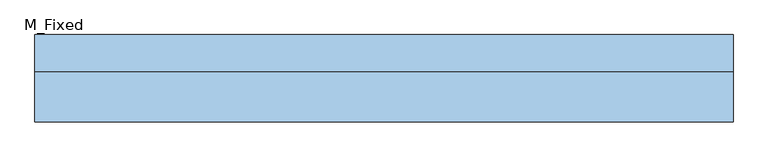
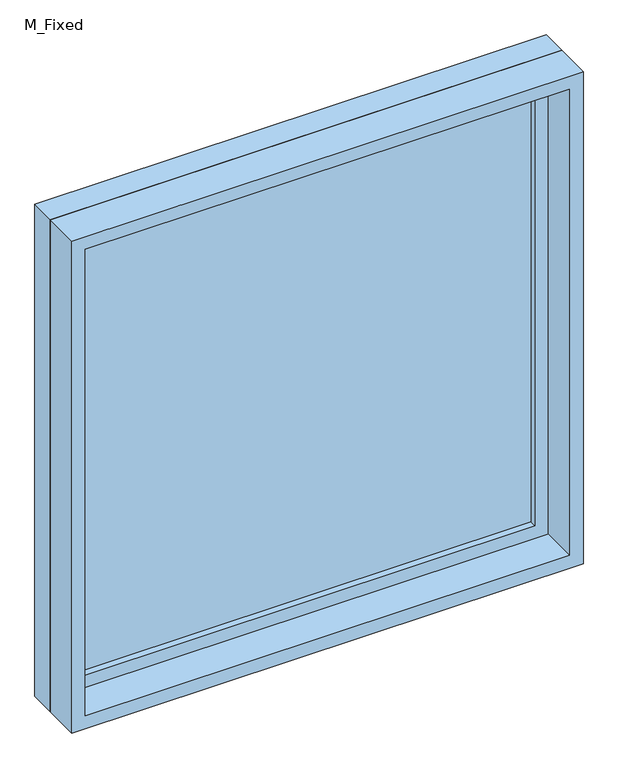
"""IFC4 building model written with IfcOpenShell, lengths in millimetres: window geometry, M_Fixed : W4 1.2 BY 1.2 M."""

from ifc_helpers import new_model, si_unit, frame, origin, place, context, project, spatial, polyline, outline, extrude, source, transform, mapped, element, save


def m_fixed_e389692a(model_context):
    return source(origin(), model_context, "Body", "SweptSolid", [
        extrude(outline(polyline([(-537.0, 53.0), (537.0, 53.0), (537.0, 41.0), (-537.0, 41.0), (-537.0, 53.0)])), frame((0.0, 0.0, 978.0), z_axis=(0.0, 0.0, 1.0), x_axis=(1.0, 0.0, 0.0)), (0.0, 0.0, 1.0), 1094.0),
        extrude(outline(polyline([(2116.0, -581.0), (934.0, -581.0), (934.0, 581.0), (2116.0, 581.0), (2116.0, -581.0)]), holes=[polyline([(2072.0, -537.0), (2072.0, 537.0), (978.0, 537.0), (978.0, -537.0), (2072.0, -537.0)])]), frame((0.0, 25.0, 0.0), z_axis=(0.0, 1.0, 0.0), x_axis=(0.0, 0.0, 1.0)), (0.0, 0.0, 1.0), 44.0),
        extrude(outline(polyline([(2135.0, -600.0), (915.0, -600.0), (915.0, 600.0), (2135.0, 600.0), (2135.0, -600.0)]), holes=[polyline([(2116.0, -581.0), (2116.0, 581.0), (934.0, 581.0), (934.0, -581.0), (2116.0, -581.0)])]), frame((0.0, 25.0, 0.0), z_axis=(0.0, 1.0, 0.0), x_axis=(0.0, 0.0, 1.0)), (0.0, 0.0, 1.0), 63.0),
        extrude(outline(polyline([(2135.0, -600.0), (915.0, -600.0), (915.0, 600.0), (2135.0, 600.0), (2135.0, -600.0)]), holes=[polyline([(2103.0, -568.0), (2103.0, 568.0), (947.0, 568.0), (947.0, -568.0), (2103.0, -568.0)])]), frame((0.0, -62.0, 0.0), z_axis=(0.0, 1.0, 0.0), x_axis=(0.0, 0.0, 1.0)), (0.0, 0.0, 1.0), 87.0),
    ])


if __name__ == "__main__":
    model = new_model("IFC4")
    model_context = context("Model", 3, world=origin())
    ifc_project = project(units=[si_unit("LENGTHUNIT", "METRE", prefix="MILLI")], contexts=[model_context])
    site = spatial("IfcSite", under=ifc_project)
    building = spatial("IfcBuilding", under=site)
    placement = place(None, origin())
    m_fixed_shape = m_fixed_e389692a(model_context)
    element("IfcWindow", 1, ObjectType="M_Fixed : W4 1.2 BY 1.2 M", at=placement, inside=building, context=model_context, shape_type="MappedRepresentation", body=[
        mapped(m_fixed_shape, transform((0.0, 0.0, 0.0), x_axis=(1.0, 0.0, 0.0), y_axis=(0.0, 1.0, 0.0), z_axis=(0.0, 0.0, 1.0))),
    ])
    save(model, "model.ifc")

# Revit data of these elements
# Type "M_Fixed : W4 1.2 BY 1.2 M"
#   Type Mark = "20"
#   Height = 1.22 m
#   Default Sill Height = 0.915 m
#   Width = 1.2 m
#   Window Inset = 0.019 m
#   Frame Exterior Material = Sash
#   Frame Interior Material = Sash
#   Glass Pane Material = Glass
#   Sash = Sash
#   Wall Closure = (empty or 0)
# Element 1 (IfcWindow, "M_Fixed : W4 1.2 BY 1.2 M")
#   Materials on its faces: "Sash", "Glass"
# Materials
#   "Sash": class "Wood", colour RGB 136 99 55, transparency 0
#   "Glass": class "Glass", colour RGB 218 227 224, transparency 0.85, Description = "Soda Lime Glass", Cost = 0
